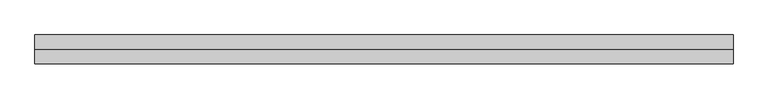
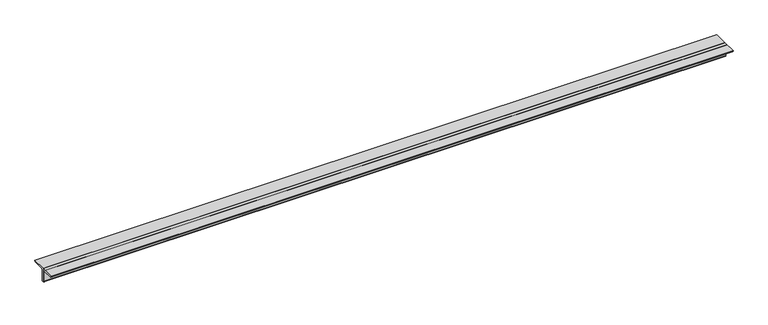
"""IFC4 building model written with IfcOpenShell, lengths in millimetres: beam geometry, 0123_Steel Framing_2Ls-KSD3502 : H_SB_AR_S04_2Ls-130x130x12_VBR2."""

from ifc_helpers import new_model, si_unit, point, frame, frame_2d, origin, place, context, project, spatial, polyline, circle_curve, trimmed, segment, composite_curve, outline, extrude, source, transform, mapped, element, save


def beam_81b2beba(model_context):
    return source(origin(), model_context, "Body", "SweptSolid", [
        extrude(outline(composite_curve([segment(polyline([(0.0, 36.4), (130.0, 36.4)]), True, "CONTINUOUS"), segment(trimmed(circle_curve(frame_2d((118.0, 36.4)), 12.0), [point((130.0, 36.4))], [point((118.0, 24.4))], False, "CARTESIAN"), True, "CONTINUOUS"), segment(polyline([(118.0, 24.4), (24.0, 24.4)]), True, "CONTINUOUS"), segment(trimmed(circle_curve(frame_2d((24.0, 12.4)), 12.0), [point((24.0, 24.4))], [point((12.0, 12.4))], True, "CARTESIAN"), True, "CONTINUOUS"), segment(polyline([(12.0, 12.4), (12.0, -81.6)]), True, "CONTINUOUS"), segment(trimmed(circle_curve(frame_2d((0.0, -81.6)), 12.0), [point((12.0, -81.6))], [point((0.0, -93.6))], False, "CARTESIAN"), True, "CONTINUOUS"), segment(polyline([(0.0, -93.6), (0.0, 36.4)]), True, "CONTINUOUS")], self_intersect=False)), frame((-3360.6041751, 0.0, 0.0), z_axis=(1.0, 0.0, 0.0), x_axis=(0.0, 1.0, 0.0)), (0.0, 0.0, 1.0), 6322.5847795),
        extrude(outline(composite_curve([segment(polyline([(0.0, 36.4), (0.0, -93.6)]), True, "CONTINUOUS"), segment(trimmed(circle_curve(frame_2d((0.0, -81.6)), 12.0), [point((0.0, -93.6))], [point((-12.0, -81.6))], False, "CARTESIAN"), True, "CONTINUOUS"), segment(polyline([(-12.0, -81.6), (-12.0, 12.4)]), True, "CONTINUOUS"), segment(trimmed(circle_curve(frame_2d((-24.0, 12.4)), 12.0), [point((-12.0, 12.4))], [point((-24.0, 24.4))], True, "CARTESIAN"), True, "CONTINUOUS"), segment(polyline([(-24.0, 24.4), (-118.0, 24.4)]), True, "CONTINUOUS"), segment(trimmed(circle_curve(frame_2d((-118.0, 36.4)), 12.0), [point((-118.0, 24.4))], [point((-130.0, 36.4))], False, "CARTESIAN"), True, "CONTINUOUS"), segment(polyline([(-130.0, 36.4), (0.0, 36.4)]), True, "CONTINUOUS")], self_intersect=False)), frame((-3360.6041751, 0.0, 0.0), z_axis=(1.0, 0.0, 0.0), x_axis=(0.0, 1.0, 0.0)), (0.0, 0.0, 1.0), 6322.5847795),
    ])


if __name__ == "__main__":
    model = new_model("IFC4")
    model_context = context("Model", 3, world=origin())
    ifc_project = project(units=[si_unit("LENGTHUNIT", "METRE", prefix="MILLI")], contexts=[model_context])
    site = spatial("IfcSite", under=ifc_project)
    building = spatial("IfcBuilding", under=site)
    placement = place(None, origin())
    beam_shape = beam_81b2beba(model_context)
    element("IfcBeam", 1, ObjectType="0123_Steel Framing_2Ls-KSD3502 : H_SB_AR_S04_2Ls-130x130x12_VBR2", at=placement, inside=building, context=model_context, shape_type="MappedRepresentation", body=[
        mapped(beam_shape, transform((0.0, 0.0, 0.0), x_axis=(1.0, 0.0, 0.0), y_axis=(0.0, 1.0, 0.0), z_axis=(0.0, 0.0, 1.0))),
    ])
    save(model, "model.ifc")

# Revit data of these elements
# Type "0123_Steel Framing_2Ls-KSD3502 : H_SB_AR_S04_2Ls-130x130x12_VBR2"
#   Type Mark = "VBR2"
#   Assembly Code = "B10"
#   Legs = "SLBB"
#   W = 8.97
#   Perimeter = 1.04 m²/m
#   Nominal Weight = 46.80 kgf/m
#   Length [instance default] = 1000 mm
#   Space = 0 mm
#   b = 130 mm
#   d = 130 mm
#   t = 12 mm
#   y = 36.4 mm
#   A = 0.005952 m²
#   Structural Material [instance default] = Steel ASTM A36
# Element 1 (IfcBeam, "0123_Steel Framing_2Ls-KSD3502 : H_SB_AR_S04_2Ls-130x130x12_VBR2")
#   Materials on its faces: "Steel ASTM A36"
# Materials
#   "Steel ASTM A36": class "Metal", colour RGB 199 199 199, transparency 0, Description = "Structural steel, ASTM A36 Grade B, mill finish", Cost = 0
